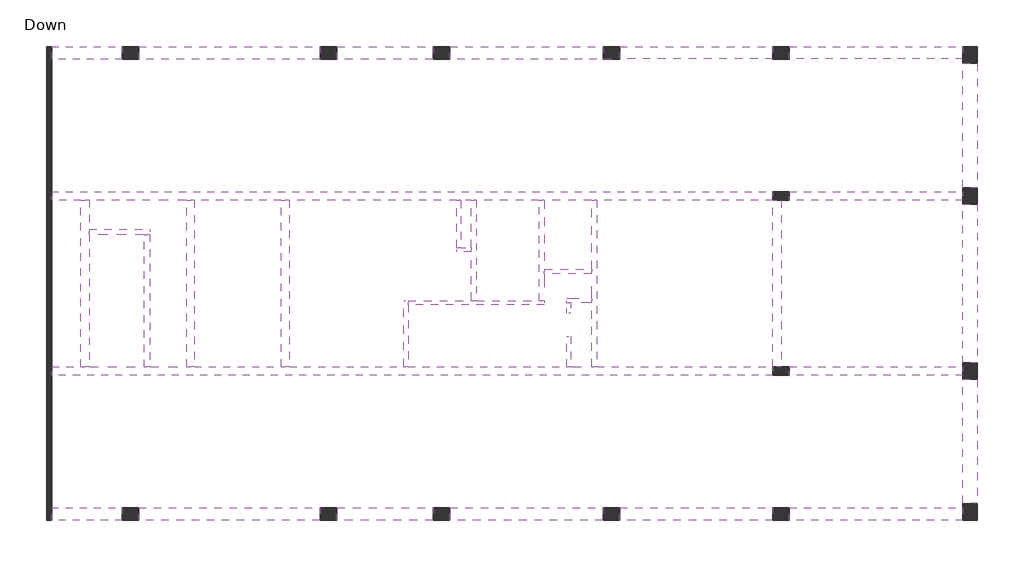
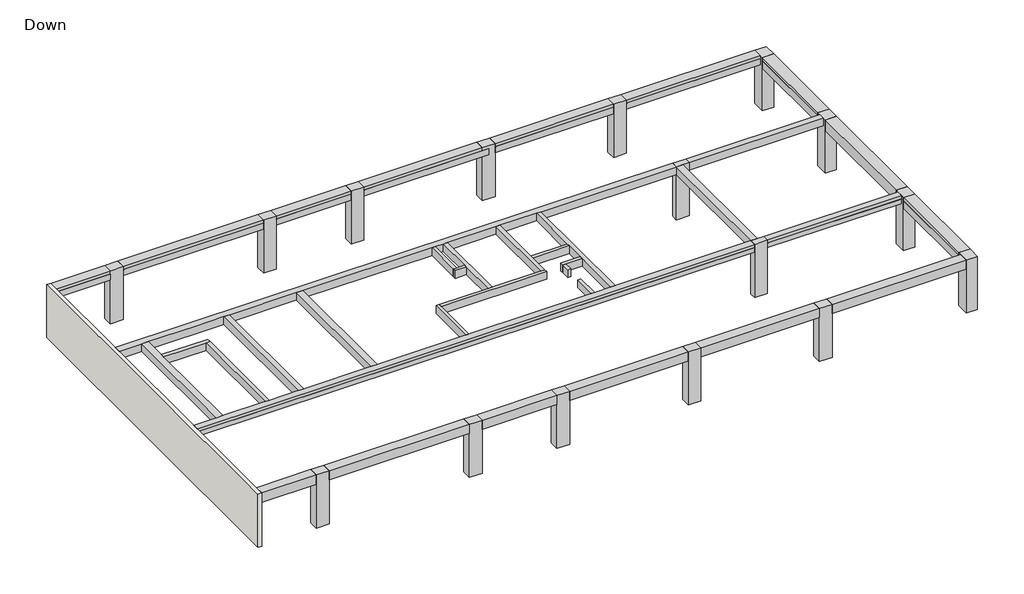
# One storey: 36 beams, 16 columns, 1 wall.
# Revit data of these elements (continued)
# Element 29 (IfcBeam, "Concrete Rectengular Beam : 60/60")
#   Comments = ""
#   Mark = "B29"
#   SOFiSTiK_AMG_Comments = ""
#   SOFiSTiK_AMG_Scheduled = yes
#   SOFiSTiK_AMG_Adjusted = yes
#   Structural Material = Concrete
#   Phase Created = New Construction
#   Materials on its faces: "Concrete"
# Element 30 (IfcBeam, "Concrete Rectengular Beam : 60/60")
#   Comments = ""
#   Mark = "B30"
#   SOFiSTiK_AMG_Comments = ""
#   SOFiSTiK_AMG_Scheduled = yes
#   SOFiSTiK_AMG_Adjusted = yes
#   Structural Material = Concrete
#   Phase Created = New Construction
#   Materials on its faces: "Concrete"
# Element 31 (IfcBeam, "Concrete Rectengular Beam : 60/60")
#   Comments = ""
#   Mark = "B31"
#   SOFiSTiK_AMG_Comments = ""
#   SOFiSTiK_AMG_Scheduled = yes
#   SOFiSTiK_AMG_Adjusted = yes
#   Structural Material = Concrete
#   Phase Created = New Construction
#   Materials on its faces: "Concrete"
# Element 32 (IfcBeam, "Concrete Rectengular Beam : 60/60")
#   Comments = ""
#   Mark = "B32"
#   SOFiSTiK_AMG_Comments = ""
#   SOFiSTiK_AMG_Scheduled = yes
#   SOFiSTiK_AMG_Adjusted = yes
#   Structural Material = Concrete
#   Phase Created = New Construction
#   Materials on its faces: "Concrete"
# Element 33 (IfcBeam, "Concrete Rectengular Beam : 60/60")
#   Comments = ""
#   Mark = "B33"
#   SOFiSTiK_AMG_Comments = ""
#   SOFiSTiK_AMG_Scheduled = yes
#   SOFiSTiK_AMG_Adjusted = yes
#   Structural Material = Concrete
#   Phase Created = New Construction
#   Materials on its faces: "Concrete"
# Element 34 (IfcBeam, "Concrete Rectengular Beam : 70/70")
#   Comments = ""
#   Mark = "B34"
#   SOFiSTiK_AMG_Comments = ""
#   SOFiSTiK_AMG_Scheduled = yes
#   SOFiSTiK_AMG_Adjusted = yes
#   Structural Material = Concrete
#   Phase Created = New Construction
#   Materials on its faces: "Concrete"
# Element 35 (IfcBeam, "Concrete Rectengular Beam : 70/70")
#   Comments = ""
#   Mark = "B35"
#   SOFiSTiK_AMG_Comments = ""
#   SOFiSTiK_AMG_Scheduled = yes
#   SOFiSTiK_AMG_Adjusted = yes
#   Structural Material = Concrete
#   Phase Created = New Construction
#   Materials on its faces: "Concrete"
# Element 36 (IfcBeam, "Concrete Rectengular Beam : 70/70")
#   Comments = ""
#   Mark = "B36"
#   SOFiSTiK_AMG_Comments = ""
#   SOFiSTiK_AMG_Scheduled = yes
#   SOFiSTiK_AMG_Adjusted = yes
#   Structural Material = Concrete
#   Phase Created = New Construction
#   Materials on its faces: "Concrete"
# Element 37 (IfcColumn, "Concrete Rectengular Column : 40/80")
#   Comments = ""
#   Mark = "C1"
#   SOFiSTiK_AMG_Comments = ""
#   SOFiSTiK_AMG_Scheduled = yes
#   SOFiSTiK_AMG_Adjusted = yes
#   Structural Material = Concrete
#   Phase Created = New Construction
#   Materials on its faces: "Concrete"
# Element 38 (IfcColumn, "Concrete Rectengular Column : 40/80")
#   Comments = ""
#   Mark = "C2"
#   SOFiSTiK_AMG_Comments = ""
#   SOFiSTiK_AMG_Scheduled = yes
#   SOFiSTiK_AMG_Adjusted = yes
#   Structural Material = Concrete
#   Phase Created = New Construction
#   Materials on its faces: "Concrete"
# Element 39 (IfcColumn, "Concrete Rectengular Column : 60/80")
#   Comments = ""
#   Mark = "C3"
#   SOFiSTiK_AMG_Comments = ""
#   SOFiSTiK_AMG_Scheduled = yes
#   SOFiSTiK_AMG_Adjusted = yes
#   Structural Material = Concrete
#   Phase Created = New Construction
#   Materials on its faces: "Concrete"
# Element 40 (IfcColumn, "Concrete Rectengular Column : 60/80")
#   Comments = ""
#   Mark = "C4"
#   SOFiSTiK_AMG_Comments = ""
#   SOFiSTiK_AMG_Scheduled = yes
#   SOFiSTiK_AMG_Adjusted = yes
#   Structural Material = Concrete
#   Phase Created = New Construction
#   Materials on its faces: "Concrete"
# Element 41 (IfcColumn, "Concrete Rectengular Column : 60/80")
#   Comments = ""
#   Mark = "C5"
#   SOFiSTiK_AMG_Comments = ""
#   SOFiSTiK_AMG_Scheduled = yes
#   SOFiSTiK_AMG_Adjusted = yes
#   Structural Material = Concrete
#   Phase Created = New Construction
#   Materials on its faces: "Concrete"
# Element 42 (IfcColumn, "Concrete Rectengular Column : 60/80")
#   Comments = ""
#   Mark = "C6"
#   SOFiSTiK_AMG_Comments = ""
#   SOFiSTiK_AMG_Scheduled = yes
#   SOFiSTiK_AMG_Adjusted = yes
#   Structural Material = Concrete
#   Phase Created = New Construction
#   Materials on its faces: "Concrete"
# Element 43 (IfcColumn, "Concrete Rectengular Column : 60/80")
#   Comments = ""
#   Mark = "C7"
#   SOFiSTiK_AMG_Comments = ""
#   SOFiSTiK_AMG_Scheduled = yes
#   SOFiSTiK_AMG_Adjusted = yes
#   Structural Material = Concrete
#   Phase Created = New Construction
#   Materials on its faces: "Concrete"
# Element 44 (IfcColumn, "Concrete Rectengular Column : 60/80")
#   Comments = ""
#   Mark = "C8"
#   SOFiSTiK_AMG_Comments = ""
#   SOFiSTiK_AMG_Scheduled = yes
#   SOFiSTiK_AMG_Adjusted = yes
#   Structural Material = Concrete
#   Phase Created = New Construction
#   Materials on its faces: "Concrete"
# Element 45 (IfcColumn, "Concrete Rectengular Column : 60/80")
#   Comments = ""
#   Mark = "C9"
#   SOFiSTiK_AMG_Comments = ""
#   SOFiSTiK_AMG_Scheduled = yes
#   SOFiSTiK_AMG_Adjusted = yes
#   Structural Material = Concrete
#   Phase Created = New Construction
#   Materials on its faces: "Concrete"
# Element 46 (IfcColumn, "Concrete Rectengular Column : 60/80")
#   Comments = ""
#   Mark = "C10"
#   SOFiSTiK_AMG_Comments = ""
#   SOFiSTiK_AMG_Scheduled = yes
#   SOFiSTiK_AMG_Adjusted = yes
#   Structural Material = Concrete
#   Phase Created = New Construction
#   Materials on its faces: "Concrete"
# Element 47 (IfcColumn, "Concrete Rectengular Column : 60/80")
#   Comments = ""
#   Mark = "C11"
#   SOFiSTiK_AMG_Comments = ""
#   SOFiSTiK_AMG_Scheduled = yes
#   SOFiSTiK_AMG_Adjusted = yes
#   Structural Material = Concrete
#   Phase Created = New Construction
#   Materials on its faces: "Concrete"
# Element 48 (IfcColumn, "Concrete Rectengular Column : 60/80")
#   Comments = ""
#   Mark = "C12"
#   SOFiSTiK_AMG_Comments = ""
#   SOFiSTiK_AMG_Scheduled = yes
#   SOFiSTiK_AMG_Adjusted = yes
#   Structural Material = Concrete
#   Phase Created = New Construction
#   Materials on its faces: "Concrete"
# Element 49 (IfcColumn, "Concrete Rectengular Column : 80/70")
#   Comments = ""
#   Mark = "C13"
#   SOFiSTiK_AMG_Comments = ""
#   SOFiSTiK_AMG_Scheduled = yes
#   SOFiSTiK_AMG_Adjusted = yes
#   Structural Material = Concrete
#   Phase Created = New Construction
#   Materials on its faces: "Concrete"
# Element 50 (IfcColumn, "Concrete Rectengular Column : 80/70")
#   Comments = ""
#   Mark = "C14"
#   SOFiSTiK_AMG_Comments = ""
#   SOFiSTiK_AMG_Scheduled = yes
#   SOFiSTiK_AMG_Adjusted = yes
#   Structural Material = Concrete
#   Phase Created = New Construction
#   Materials on its faces: "Concrete"
# Element 51 (IfcColumn, "Concrete Rectengular Column : 80/70")
#   Comments = ""
#   Mark = "C15"
#   SOFiSTiK_AMG_Comments = ""
#   SOFiSTiK_AMG_Scheduled = yes
#   SOFiSTiK_AMG_Adjusted = yes
#   Structural Material = Concrete
#   Phase Created = New Construction
#   Materials on its faces: "Concrete"
# Element 52 (IfcColumn, "Concrete Rectengular Column : 80/70")
#   Comments = ""
#   Mark = "C16"
#   SOFiSTiK_AMG_Comments = ""
#   SOFiSTiK_AMG_Scheduled = yes
#   SOFiSTiK_AMG_Adjusted = yes
#   Structural Material = Concrete
#   Phase Created = New Construction
#   Materials on its faces: "Concrete"
# Element 53 (IfcWall, "25")
#   Comments = ""
#   Mark = "W1"
#   SOFiSTiK_EdgeZones = "W1"
#   SOFiSTiK_AMG_Comments = ""
#   Top Offset = 0 cm
#   Base Offset = 0 cm
#   wall height = 350 cm
#   SOFiSTiK_AMG_Scheduled = yes
#   SOFiSTiK_AMG_Adjusted = yes
#   Phase Created = New Construction
#   Base Constraint = Down
#   Top Constraint = Typical Floor
#   Materials on its faces: "Concrete"
# Materials
#   "Concrete": class "Concrete", colour RGB 192 192 192, transparency 0, Keynote = "01000", Description = "Cast-in-place concrete", Cost = 0
